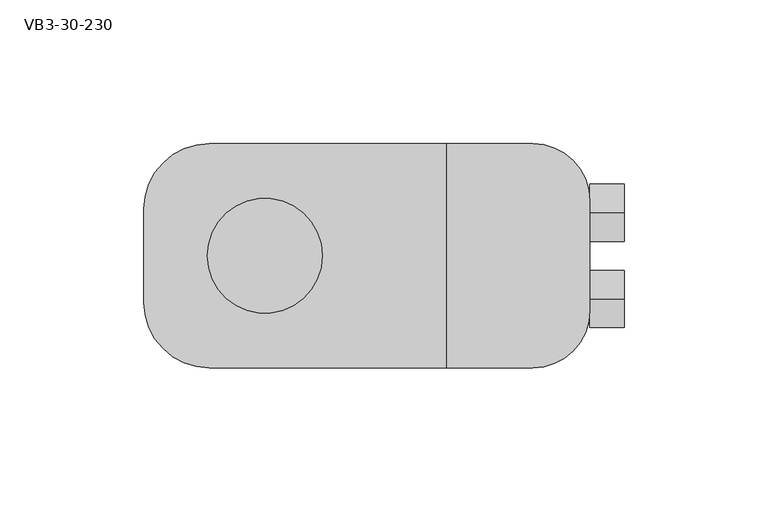
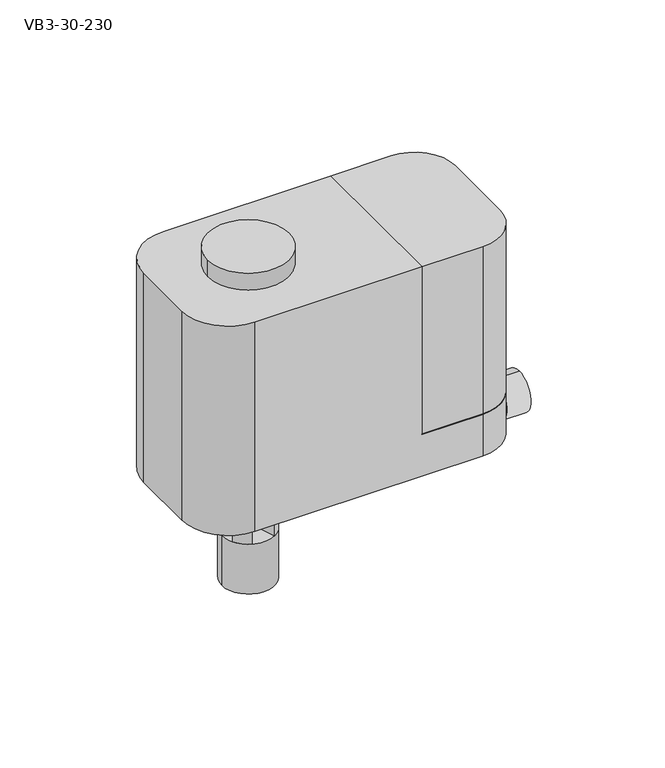
"""IFC4 building model written with IfcOpenShell, lengths in millimetres: proxy geometry, electroprivod_vb3_vba3-30 : VB3-30-230."""

import ifcopenshell
import ifcopenshell.guid

model = None  # the IFC model being written
_history = None  # IfcOwnerHistory: only IFC2X3 demands one
_inside = {}  # id of a spatial element -> (the spatial element, [elements in it])
_under = {}  # id of a project, library or spatial element -> (it, [spatial elements below it])
_declared = {}  # id of a project -> (the project, [libraries it declares])
_typed = {}  # id of a type object -> (the type object, [elements of that type])
_made_of = {}  # id of a material, layer set ... -> (it, [elements and type objects made of it])


def new_model(schema):
    """Start an empty IFC model of exactly this schema.

    Asked for "IFC4X3", IfcOpenShell would pick the latest addendum, in which some entities
    have other attributes; the version numbers below select the first issue.
    IFC2X3 requires an IfcOwnerHistory on every rooted entity: one is made here for all.
    """
    global model, _history
    if schema == "IFC4X3":
        model = ifcopenshell.file(schema_version=(4, 3, 0, 0))
    else:
        model = ifcopenshell.file(schema=schema)
    _inside.clear()
    _under.clear()
    _declared.clear()
    _typed.clear()
    _made_of.clear()
    _history = None
    if model.schema == "IFC2X3":
        org = make("IfcOrganization", Name="unknown")
        user = make(
            "IfcPersonAndOrganization",
            ThePerson=make("IfcPerson", FamilyName="unknown"),
            TheOrganization=org,
        )
        app = make(
            "IfcApplication",
            ApplicationDeveloper=org,
            Version="unknown",
            ApplicationFullName="unknown",
            ApplicationIdentifier="unknown",
        )
        _history = make(
            "IfcOwnerHistory",
            OwningUser=user,
            OwningApplication=app,
            ChangeAction="ADDED",
            CreationDate=0,
        )
    return model


def make(cls, **values):
    """One entity of the class cls with the attributes given. An attribute that is None is left unset."""
    return model.create_entity(
        cls, **{name: value for name, value in values.items() if value is not None}
    )


def rooted(cls, **values):
    """An entity with a GlobalId (a new one), such as an element, a storey or a relation."""
    return make(cls, GlobalId=ifcopenshell.guid.new(), OwnerHistory=_history, **values)


def si_unit(unit_type, name, prefix=None):
    """IfcSIUnit, for example si_unit("LENGTHUNIT", "METRE", prefix="MILLI")."""
    return make("IfcSIUnit", UnitType=unit_type, Prefix=prefix, Name=name)


def assignment(units):
    """IfcUnitAssignment: the units of a project."""
    return None if units is None else make("IfcUnitAssignment", Units=units)


def point(xyz):
    """IfcCartesianPoint."""
    return None if xyz is None else make("IfcCartesianPoint", Coordinates=xyz)


def direction(xyz):
    """IfcDirection."""
    return None if xyz is None else make("IfcDirection", DirectionRatios=xyz)


def frame(location, z_axis=None, x_axis=None):
    """IfcAxis2Placement3D, a coordinate frame: its origin and axes. An axis left out is left unset."""
    return make(
        "IfcAxis2Placement3D",
        Location=point(location),
        Axis=direction(z_axis),
        RefDirection=direction(x_axis),
    )


def frame_2d(location, x_axis=None):
    """IfcAxis2Placement2D, a coordinate frame in the plane: its origin and x axis."""
    return make(
        "IfcAxis2Placement2D", Location=point(location), RefDirection=direction(x_axis)
    )


def origin():
    """The frame at (0, 0, 0) with its axes left unset."""
    return frame((0.0, 0.0, 0.0))


def origin_with_axes():
    """The frame at (0, 0, 0) with the z axis (0, 0, 1) and the x axis (1, 0, 0) written out."""
    return frame((0.0, 0.0, 0.0), z_axis=(0.0, 0.0, 1.0), x_axis=(1.0, 0.0, 0.0))


def origin_2d():
    """The frame at (0, 0) in the plane with its x axis left unset."""
    return frame_2d((0.0, 0.0))


def place(relative_to, where):
    """IfcLocalPlacement: puts the frame where relative to a parent placement (None: the world)."""
    return make(
        "IfcLocalPlacement", PlacementRelTo=relative_to, RelativePlacement=where
    )


def context(
    kind, dimensions, precision=None, world=None, true_north=None, identifier=None
):
    """IfcGeometricRepresentationContext, for example the 3D "Model" context."""
    return make(
        "IfcGeometricRepresentationContext",
        ContextIdentifier=identifier,
        ContextType=kind,
        CoordinateSpaceDimension=dimensions,
        Precision=precision,
        WorldCoordinateSystem=world,
        TrueNorth=true_north,
    )


def project(units=None, contexts=None):
    """IfcProject with its units and contexts."""
    return rooted(
        "IfcProject",
        Name="project",
        RepresentationContexts=contexts,
        UnitsInContext=assignment(units),
    )


def spatial(cls, under=None, at=None, **own):
    """A site, building, storey or space (cls), placed at a placement, below another one or the project."""
    s = rooted(cls, ObjectPlacement=at, **own)
    if under is not None:
        _under.setdefault(under.id(), (under, []))[1].append(s)
    return s


def polyline(points):
    """IfcPolyline through the points."""
    return make("IfcPolyline", Points=[point(p) for p in points])


def circle_curve(where, radius):
    """IfcCircle in the frame where."""
    return make("IfcCircle", Position=where, Radius=radius)


def trimmed(basis, trim1, trim2, sense, master):
    """IfcTrimmedCurve: the piece of a basis curve between two trims."""
    return make(
        "IfcTrimmedCurve",
        BasisCurve=basis,
        Trim1=trim1,
        Trim2=trim2,
        SenseAgreement=sense,
        MasterRepresentation=master,
    )


def segment(curve, same_sense, transition):
    """IfcCompositeCurveSegment."""
    return make(
        "IfcCompositeCurveSegment",
        Transition=transition,
        SameSense=same_sense,
        ParentCurve=curve,
    )


def composite_curve(segments, self_intersect=None):
    """IfcCompositeCurve: segments joined end to end."""
    return make("IfcCompositeCurve", Segments=segments, SelfIntersect=self_intersect)


def outline(outer, holes=None, kind="AREA"):
    """IfcArbitraryClosedProfileDef: a profile drawn as a closed curve; with holes, ...WithVoids."""
    if holes is None:
        return make("IfcArbitraryClosedProfileDef", ProfileType=kind, OuterCurve=outer)
    return make(
        "IfcArbitraryProfileDefWithVoids",
        ProfileType=kind,
        OuterCurve=outer,
        InnerCurves=holes,
    )


def extrude(swept, where, along, depth):
    """IfcExtrudedAreaSolid: the profile swept, set in the frame where, extruded along a direction by depth."""
    return make(
        "IfcExtrudedAreaSolid",
        SweptArea=swept,
        Position=where,
        ExtrudedDirection=direction(along),
        Depth=depth,
    )


def shape(context_of_items, identifier, shape_type, items):
    """IfcShapeRepresentation: the items that make up one representation, for example the "Body"."""
    return make(
        "IfcShapeRepresentation",
        ContextOfItems=context_of_items,
        RepresentationIdentifier=identifier,
        RepresentationType=shape_type,
        Items=items,
    )


def source(mapping_origin, context_of_items, identifier, shape_type, items):
    """IfcRepresentationMap: a shape defined once, which mapped items show again and again."""
    return make(
        "IfcRepresentationMap",
        MappingOrigin=mapping_origin,
        MappedRepresentation=shape(context_of_items, identifier, shape_type, items),
    )


def transform(
    local_origin,
    x_axis=None,
    y_axis=None,
    z_axis=None,
    scale=None,
    scale2=None,
    scale3=None,
    uniform=True,
):
    """IfcCartesianTransformationOperator3D, or its non-uniform kind. x_axis, y_axis, z_axis: its Axis1, 2, 3."""
    if uniform:
        return make(
            "IfcCartesianTransformationOperator3D",
            Axis1=direction(x_axis),
            Axis2=direction(y_axis),
            LocalOrigin=point(local_origin),
            Scale=scale,
            Axis3=direction(z_axis),
        )
    return make(
        "IfcCartesianTransformationOperator3DnonUniform",
        Axis1=direction(x_axis),
        Axis2=direction(y_axis),
        LocalOrigin=point(local_origin),
        Scale=scale,
        Axis3=direction(z_axis),
        Scale2=scale2,
        Scale3=scale3,
    )


def mapped(mapping_source, mapping_target):
    """IfcMappedItem: shows the shape of a source again, moved by a transform."""
    return make(
        "IfcMappedItem", MappingSource=mapping_source, MappingTarget=mapping_target
    )


def made_of(thing, what):
    """Note that an element or type object is made of a material, layer set ...; save() writes the relation."""
    if what is not None:
        _made_of.setdefault(what.id(), (what, []))[1].append(thing)
    return thing


def element(
    cls,
    number,
    at=None,
    inside=None,
    cuts=None,
    type_object=None,
    material=None,
    context=None,
    identifier="Body",
    shape_type=None,
    held_by="IfcProductDefinitionShape",
    body=None,
    shapes=None,
    **own,
):
    """One element of the class cls, such as IfcWall. Its Tag is "e" and its number.

    at: its placement. inside: the storey or other place that contains it. cuts: it is an
    opening in that element (IfcRelVoidsElement). A single representation is given by context,
    identifier, shape_type and body (its items); several are given by shapes. held_by: the class
    of the entity that holds the representations. save() writes the other relations.
    """
    e = rooted(cls, Tag="e%d" % number, ObjectPlacement=at, **own)
    if body is not None:
        shapes = [shape(context, identifier, shape_type, body)]
    if shapes is not None:
        e.Representation = make(held_by, Representations=shapes)
    if inside is not None:
        _inside.setdefault(inside.id(), (inside, []))[1].append(e)
    if cuts is not None:
        rooted(
            "IfcRelVoidsElement", RelatingBuildingElement=cuts, RelatedOpeningElement=e
        )
    if type_object is not None:
        _typed.setdefault(type_object.id(), (type_object, []))[1].append(e)
    return made_of(e, material)


def aggregate(whole, parts):
    """IfcRelAggregates: a whole, such as a stair, and the parts it consists of."""
    return rooted("IfcRelAggregates", RelatingObject=whole, RelatedObjects=parts)


def save(model, path):
    """Write the relations noted so far, then the file.

    IfcRelAggregates (storeys below a building ...), IfcRelContainedInSpatialStructure (elements
    in a storey), IfcRelDefinesByType, IfcRelAssociatesMaterial and IfcRelDeclares: one each for
    every whole, place, type object, material and project.
    """
    for whole, parts in _under.values():
        aggregate(whole, parts)
    for where, things in _inside.values():
        rooted(
            "IfcRelContainedInSpatialStructure",
            RelatedElements=things,
            RelatingStructure=where,
        )
    for kind, things in _typed.values():
        rooted("IfcRelDefinesByType", RelatedObjects=things, RelatingType=kind)
    for what, things in _made_of.values():
        rooted("IfcRelAssociatesMaterial", RelatedObjects=things, RelatingMaterial=what)
    for by, libraries in _declared.values():
        rooted("IfcRelDeclares", RelatingContext=by, RelatedDefinitions=libraries)
    model.write(path)


def plane_surface(at):
    """IfcPlane: the flat surface through the origin of the frame at, square to its z axis."""
    return make("IfcPlane", Position=at)


def cylinder_surface(at, radius):
    """IfcCylindricalSurface: all points at the distance radius from the z axis of the frame at."""
    return make("IfcCylindricalSurface", Position=at, Radius=radius)


def advanced_brep(points, edges, surfaces, faces):
    """IfcAdvancedBrep: a solid bounded by faces that lie on surfaces and meet in shared edges.

    An edge is (start, end): straight between two places in points (the first is 0);
    or (start, end, curve); or (start, end, curve, False) where it runs against its curve.
    A face is (place in surfaces, loops), or (place, loops, False) where it looks against
    its surface's normal. A loop lists edges by number (the first is 1), with a minus sign
    where the edge is run from its end to its start. The first loop is the outer one.
    """
    corners = [point(p) for p in points]
    vertices = [make("IfcVertexPoint", VertexGeometry=c) for c in corners]
    made = []
    for start, end, *more in edges:
        made.append(
            make(
                "IfcEdgeCurve",
                EdgeStart=vertices[start],
                EdgeEnd=vertices[end],
                EdgeGeometry=more[0] if more else make("IfcPolyline", Points=[corners[start], corners[end]]),
                SameSense=more[1] if len(more) > 1 else True,
            )
        )
    hull = []
    for where, loops, *sense in faces:
        bounds = []
        for j, loop in enumerate(loops):
            ring = [make("IfcOrientedEdge", EdgeElement=made[abs(k) - 1], Orientation=k > 0) for k in loop]
            bounds.append(
                make(
                    "IfcFaceOuterBound" if j == 0 else "IfcFaceBound",
                    Bound=make("IfcEdgeLoop", EdgeList=ring),
                    Orientation=True,
                )
            )
        hull.append(make("IfcAdvancedFace", Bounds=bounds, FaceSurface=surfaces[where], SameSense=sense[0] if sense else True))
    return make("IfcAdvancedBrep", Outer=make("IfcClosedShell", CfsFaces=hull))


def vb3_30_230_b1ec5a9c(model_context):
    return source(origin(), model_context, "Body", "SolidModel", [
        advanced_brep(
        [(63.0471136, 39.0, 163.0), (-19.2931357, 39.0, 163.0), (-42.0814606, 16.2116751, 163.0), (-42.0814606, -16.2116751, 163.0), (-19.2931357, -39.0, 163.0), (63.0471136, -39.0, 163.0), (-42.0814606, 16.2116751, 54.0), (-42.0814606, -16.2116751, 54.0), (63.0471136, -39.0, 75.6666667), (63.0471136, 39.0, 75.6666667), (-19.2931357, 39.0, 54.0), (-19.2931357, -39.0, 54.0), (93.0471136, -39.0, 75.6666667), (113.0, -19.0471136, 75.6666667), (113.0, 19.0471136, 75.6666667), (93.0471136, 39.0, 75.6666667), (93.0471136, 39.0, 54.0), (113.0, 19.0471136, 54.0), (113.0, -19.0471136, 54.0), (93.0471136, -39.0, 54.0)],
        [
            (0, 1),
            (1, 2, circle_curve(frame((-19.2931357, 16.2116751, 163.0), z_axis=(0.0, 0.0, 1.0), x_axis=(1.0, 0.0, 0.0)), 22.7883249)),
            (2, 3),
            (3, 4, circle_curve(frame((-19.2931357, -16.2116751, 163.0), z_axis=(0.0, 0.0, 1.0), x_axis=(1.0, 0.0, 0.0)), 22.7883249)),
            (4, 5),
            (5, 0),
            (2, 6),
            (6, 7),
            (7, 3),
            (5, 8),
            (8, 9),
            (9, 0),
            (1, 10),
            (10, 6, circle_curve(frame((-19.2931357, 16.2116751, 54.0), z_axis=(0.0, 0.0, 1.0), x_axis=(1.0, 0.0, 0.0)), 22.7883249)),
            (7, 11, circle_curve(frame((-19.2931357, -16.2116751, 54.0), z_axis=(0.0, 0.0, 1.0), x_axis=(1.0, 0.0, 0.0)), 22.7883249)),
            (11, 4),
            (8, 12),
            (12, 13, circle_curve(frame((93.0471136, -19.0471136, 75.6666667), z_axis=(0.0, 0.0, 1.0), x_axis=(1.0, 0.0, 0.0)), 19.9528864)),
            (13, 14),
            (14, 15, circle_curve(frame((93.0471136, 19.0471136, 75.6666667), z_axis=(0.0, 0.0, 1.0), x_axis=(1.0, 0.0, 0.0)), 19.9528864)),
            (15, 9),
            (16, 17, circle_curve(frame((93.0471136, 19.0471136, 54.0), z_axis=(0.0, 0.0, -1.0), x_axis=(1.0, 0.0, 0.0)), 19.9528864)),
            (17, 18),
            (18, 19, circle_curve(frame((93.0471136, -19.0471136, 54.0), z_axis=(0.0, 0.0, -1.0), x_axis=(1.0, 0.0, 0.0)), 19.9528864)),
            (19, 11),
            (10, 16),
            (19, 12),
            (18, 13),
            (17, 14),
            (16, 15),
        ],
        [
            plane_surface(frame((-19.2931357, 39.0, 163.0), z_axis=(0.0, 0.0, 1.0), x_axis=(-1.0, 0.0, 0.0))),
            plane_surface(frame((-42.0814606, 16.2116751, 163.0), z_axis=(-1.0, 0.0, 0.0), x_axis=(0.0, 0.0, -1.0))),
            plane_surface(frame((63.0471136, -39.0, 163.0), z_axis=(1.0, 0.0, 0.0), x_axis=(0.0, 0.0, -1.0))),
            cylinder_surface(frame((-19.2931357, 16.2116751, 54.0), z_axis=(0.0, 0.0, 1.0), x_axis=(1.0, 0.0, 0.0)), 22.7883249),
            cylinder_surface(frame((-19.2931357, -16.2116751, 54.0), z_axis=(0.0, 0.0, 1.0), x_axis=(1.0, 0.0, 0.0)), 22.7883249),
            plane_surface(frame((63.0471136, -39.0, 75.6666667), z_axis=(0.0, 0.0, 1.0), x_axis=(1.0, 0.0, 0.0))),
            plane_surface(frame((63.0471136, -39.0, 54.0), z_axis=(0.0, 0.0, -1.0), x_axis=(-1.0, 0.0, 0.0))),
            plane_surface(frame((63.0471136, -39.0, 75.6666667), z_axis=(0.0, -1.0, 0.0), x_axis=(0.0, 0.0, -1.0))),
            cylinder_surface(frame((93.0471136, -19.0471136, 54.0), z_axis=(0.0, 0.0, 1.0), x_axis=(1.0, 0.0, 0.0)), 19.9528864),
            plane_surface(frame((113.0, -19.0471136, 75.6666667), z_axis=(1.0, 0.0, 0.0), x_axis=(0.0, 0.0, -1.0))),
            cylinder_surface(frame((93.0471136, 19.0471136, 54.0), z_axis=(0.0, 0.0, 1.0), x_axis=(1.0, 0.0, 0.0)), 19.9528864),
            plane_surface(frame((93.0471136, 39.0, 75.6666667), z_axis=(0.0, 1.0, 0.0), x_axis=(0.0, 0.0, -1.0))),
        ],
        [
            (0, [[1, 2, 3, 4, 5, 6]]),
            (1, [[-3, 7, 8, 9]]),
            (2, [[-6, 10, 11, 12]]),
            (3, [[-2, 13, 14, -7]]),
            (4, [[-4, -9, 15, 16]]),
            (5, [[17, 18, 19, 20, 21, -11]]),
            (6, [[22, 23, 24, 25, -15, -8, -14, 26]]),
            (7, [[-17, -10, -5, -16, -25, 27]]),
            (8, [[-18, -27, -24, 28]]),
            (9, [[-19, -28, -23, 29]]),
            (10, [[-20, -29, -22, 30]]),
            (11, [[-21, -30, -26, -13, -1, -12]]),
        ],
    ),
        extrude(outline(composite_curve([segment(trimmed(circle_curve(origin_2d(), 13.0), [point((-5.0827807, -11.965172))], [point((-11.3955298, -6.2563489))], False, "CARTESIAN"), True, "CONTINUOUS"), segment(polyline([(-11.3955298, -6.2563489), (-2.9774493, -3.5211488), (-5.0827807, -11.965172)]), True, "CONTINUOUS")], self_intersect=False)), frame((0.0, 0.0, 26.0), z_axis=(0.0, 0.0, 1.0), x_axis=(1.0, 0.0, 0.0)), (0.0, 0.0, 1.0), 28.0),
        extrude(outline(composite_curve([segment(trimmed(circle_curve(origin_2d(), 13.0), [point((11.4744221, -6.1104531))], [point((6.3527375, -11.3420777))], False, "CARTESIAN"), True, "CONTINUOUS"), segment(polyline([(6.3527375, -11.3420777), (3.5062581, -3.5214397), (11.4744221, -6.1104531)]), True, "CONTINUOUS")], self_intersect=False)), frame((0.0, 0.0, 26.0), z_axis=(0.0, 0.0, 1.0), x_axis=(1.0, 0.0, 0.0)), (0.0, 0.0, 1.0), 28.0),
        extrude(outline(composite_curve([segment(trimmed(circle_curve(origin_2d(), 13.0), [point((-12.2082792, 4.4674288))], [point((-7.5582211, 10.5770172))], False, "CARTESIAN"), True, "CONTINUOUS"), segment(polyline([(-7.5582211, 10.5770172), (-5.125779, 3.0907302), (-12.2082792, 4.4674288)]), True, "CONTINUOUS")], self_intersect=False)), frame((0.0, 0.0, 26.0), z_axis=(0.0, 0.0, 1.0), x_axis=(1.0, 0.0, 0.0)), (0.0, 0.0, 1.0), 28.0),
        extrude(outline(composite_curve([segment(trimmed(circle_curve(origin_2d(), 13.0), [point((8.7963668, 9.572039))], [point((12.0714677, 4.8249007))], False, "CARTESIAN"), True, "CONTINUOUS"), segment(polyline([(12.0714677, 4.8249007), (6.2966743, 3.385083), (8.7963668, 9.572039)]), True, "CONTINUOUS")], self_intersect=False)), frame((0.0, 0.0, 26.0), z_axis=(0.0, 0.0, 1.0), x_axis=(1.0, 0.0, 0.0)), (0.0, 0.0, 1.0), 28.0),
        extrude(outline(composite_curve([segment(trimmed(circle_curve(origin_2d(), 13.0), [point((-13.0, 0.0))], [point((13.0, 0.0))], False, "CARTESIAN"), True, "CONTINUOUS"), segment(trimmed(circle_curve(origin_2d(), 13.0), [point((13.0, 0.0))], [point((-13.0, 0.0))], False, "CARTESIAN"), True, "CONTINUOUS")], self_intersect=False)), origin_with_axes(), (0.0, 0.0, 1.0), 26.0),
        extrude(outline(composite_curve([segment(trimmed(circle_curve(frame_2d((15.0, 62.5510492)), 10.0), [point((15.0, 52.5510492))], [point((15.0, 72.5510492))], False, "CARTESIAN"), True, "CONTINUOUS"), segment(trimmed(circle_curve(frame_2d((15.0, 62.5510492)), 10.0), [point((15.0, 72.5510492))], [point((15.0, 52.5510492))], False, "CARTESIAN"), True, "CONTINUOUS")], self_intersect=False)), frame((113.0, 0.0, 0.0), z_axis=(1.0, 0.0, 0.0), x_axis=(0.0, 1.0, 0.0)), (0.0, 0.0, 1.0), 11.9185394),
        extrude(outline(composite_curve([segment(trimmed(circle_curve(frame_2d((-15.0, 62.5510492)), 10.0), [point((-15.0, 52.5510492))], [point((-15.0, 72.5510492))], False, "CARTESIAN"), True, "CONTINUOUS"), segment(trimmed(circle_curve(frame_2d((-15.0, 62.5510492)), 10.0), [point((-15.0, 72.5510492))], [point((-15.0, 52.5510492))], False, "CARTESIAN"), True, "CONTINUOUS")], self_intersect=False)), frame((113.0, 0.0, 0.0), z_axis=(1.0, 0.0, 0.0), x_axis=(0.0, 1.0, 0.0)), (0.0, 0.0, 1.0), 11.9185394),
        extrude(outline(composite_curve([segment(trimmed(circle_curve(origin_2d(), 20.0), [point((-20.0, 0.0))], [point((20.0, 0.0))], False, "CARTESIAN"), True, "CONTINUOUS"), segment(trimmed(circle_curve(origin_2d(), 20.0), [point((20.0, 0.0))], [point((-20.0, 0.0))], False, "CARTESIAN"), True, "CONTINUOUS")], self_intersect=False)), frame((0.0, 0.0, 163.0), z_axis=(0.0, 0.0, 1.0), x_axis=(1.0, 0.0, 0.0)), (0.0, 0.0, 1.0), 9.0),
        extrude(outline(composite_curve([segment(trimmed(circle_curve(frame_2d((93.0471136, -19.0471136)), 19.9528864), [point((113.0, -19.0471136))], [point((93.0471136, -39.0))], False, "CARTESIAN"), True, "CONTINUOUS"), segment(polyline([(93.0471136, -39.0), (63.0471136, -39.0), (63.0471136, 39.0), (93.0471136, 39.0)]), True, "CONTINUOUS"), segment(trimmed(circle_curve(frame_2d((93.0471136, 19.0471136)), 19.9528864), [point((93.0471136, 39.0))], [point((113.0, 19.0471136))], False, "CARTESIAN"), True, "CONTINUOUS"), segment(polyline([(113.0, 19.0471136), (113.0, -19.0471136)]), True, "CONTINUOUS")], self_intersect=False)), frame((0.0, 0.0, 75.6666667), z_axis=(0.0, 0.0, 1.0), x_axis=(1.0, 0.0, 0.0)), (0.0, 0.0, 1.0), 87.3333333),
    ])


if __name__ == "__main__":
    model = new_model("IFC4")
    model_context = context("Model", 3, world=origin())
    ifc_project = project(units=[si_unit("LENGTHUNIT", "METRE", prefix="MILLI")], contexts=[model_context])
    site = spatial("IfcSite", under=ifc_project)
    building = spatial("IfcBuilding", under=site)
    placement = place(None, origin())
    vb3_30_230_shape = vb3_30_230_b1ec5a9c(model_context)
    element("IfcBuildingElementProxy", 1, Name="electroprivod_vb3_vba3-30 : VB3-30-230", ObjectType="electroprivod_vb3_vba3-30 : VB3-30-230", at=placement, inside=building, context=model_context, shape_type="MappedRepresentation", body=[
        mapped(vb3_30_230_shape, transform((0.0, 0.0, 0.0), x_axis=(1.0, 0.0, 0.0), y_axis=(0.0, 1.0, 0.0), z_axis=(0.0, 0.0, 1.0))),
    ])
    save(model, "model.ifc")

# Revit data of these elements
# Type "electroprivod_vb3_vba3-30 : VB3-30-230"
#   Усилие = "300H+30%"
#   Степень защиты = "IP 54"
#   Разработано = "support@bimlib.ru"
#   Watermarked By = ""
#   Manufacturer = "Broen"
#   Диапазон температур = "-5°C ...+55°C"
#   Входной сигнал = "Трехпозиционный"
#   Время закрытия/открытия = "33/66"
#   URL = "https://broen.ru/"
#   FL_Таблица4 = "VB3-30-DN"
#   FL_Таблица1 = "VB3-30-Наименование"
#   FL_Таблица3 = "VB3-30-Артикул"
#   FL_Таблица2 = "VB3-30-Обозначение"
#   DN [instance default] = "65"
#   ADSK_Примечание [instance default] = ""
#   ADSK_Позиция [instance default] = ""
#   ADSK_Обозначение [instance default] = "VB3-30-230."
#   ADSK_Наименование [instance default] = "Электропривод регулирующий VB3-30-230."
#   ADSK_Масса_Текст [instance default] = "0,7"
#   ADSK_Марка [instance default] = "VB3-30-230."
#   ADSK_Код изделия [instance default] = "1-5220100"
#   ADSK_Завод-изготовитель = "Broen"
#   ADSK_Единица измерения = "шт."
#   ADSK_URL страницы изделия = "https://broen.ru/product_clorius.php?info=30"
#   ADSK_URL документации изделия = "https://broen.ru/media/Directory_of_Regulating-and_stop-valves_03_2018.pdf"
#   Частота = 50 Hz
#   Ход штока = 11 mm
#   Default Elevation = 1219.2 mm
#   Напряжение = 230 V
#   Коннектор высота = 63 mm
#   Коннектор центр = 30 mm
#   Коннектор справа = 125 mm
#   Потребляемая мощность = 3 W
#   A [instance default] = 172 mm
#   C [instance default] = 133 mm
#   B [instance default] = 159 mm
#   D [instance default] = 26 mm
#   ADSK_Расход жидкости = 0.0 L/s
#   ADSK_Полная мощность = 0 VA
#   ADSK_Масса [instance default] = 0.7
#   код = 1
#   ADSK_Количество фаз = 1
#   3 фазный = yes
#   Тип Клапана = element 1328511
#   Клапан3 = element 1328512
#   Клапан1 = element 1328511
#   Материал корпуса = Алюминиевый сплав
#   Материал компонентов = Нержавеющая cталь
# Element 1 (IfcBuildingElementProxy, "electroprivod_vb3_vba3-30 : VB3-30-230")
#   Materials on its faces: "Алюминиевый сплав", "Нержавеющая cталь", "Стекло"
# Materials
#   "Алюминиевый сплав": class "Металл", colour RGB 120 120 120, transparency 0, Keynote = "﻿﻿             ﻿     ﻿                                                          ﻿   ​ ﻿                   ﻿          ​       ﻿  ﻿     ﻿   ​  ﻿  ﻿ ﻿          ﻿       ​          ​       ​ ​ ﻿﻿", Comments = "﻿﻿             ﻿     ﻿                                                          ﻿   ​ ﻿                   ﻿          ​       ﻿  ﻿     ﻿   ​  ﻿  ﻿ ﻿          ﻿       ​          ​       ​ ​ ﻿﻿", Description = "Anodized aluminum, red", Cost = 0
#   "Нержавеющая cталь": class "Металл", colour RGB 120 120 120, transparency 0, Keynote = "﻿﻿             ﻿     ﻿                                                          ﻿   ​ ﻿                   ﻿          ​       ﻿  ﻿     ﻿   ​  ﻿  ﻿ ﻿          ﻿       ​          ​       ​ ​ ﻿﻿", Comments = "﻿﻿             ﻿     ﻿                                                          ﻿   ​ ﻿                   ﻿          ​       ﻿  ﻿     ﻿   ​  ﻿  ﻿ ﻿          ﻿       ​          ​       ​ ​ ﻿﻿", Description = "Сталь нержавеющая", Cost = 0
#   "Стекло": class "Стекло", colour RGB 0 0 255, transparency 0.75, Cost = 0
